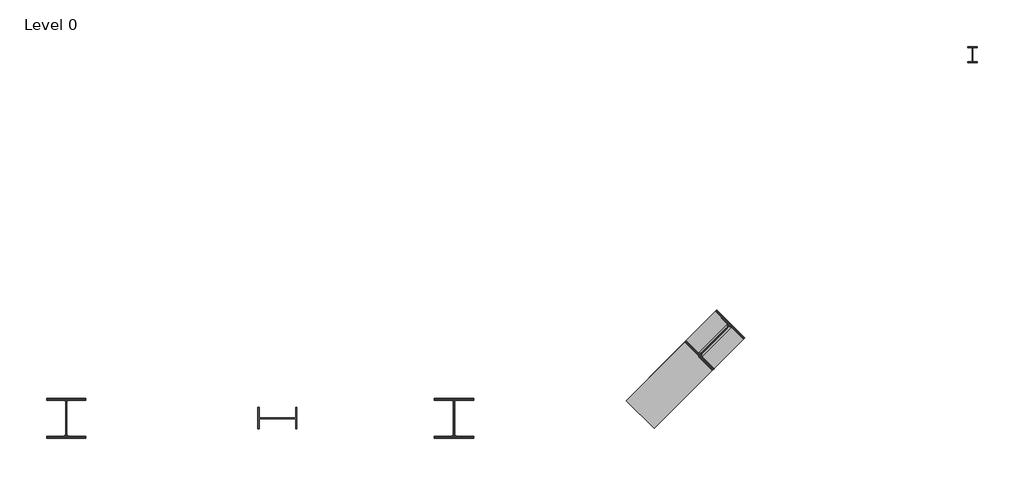
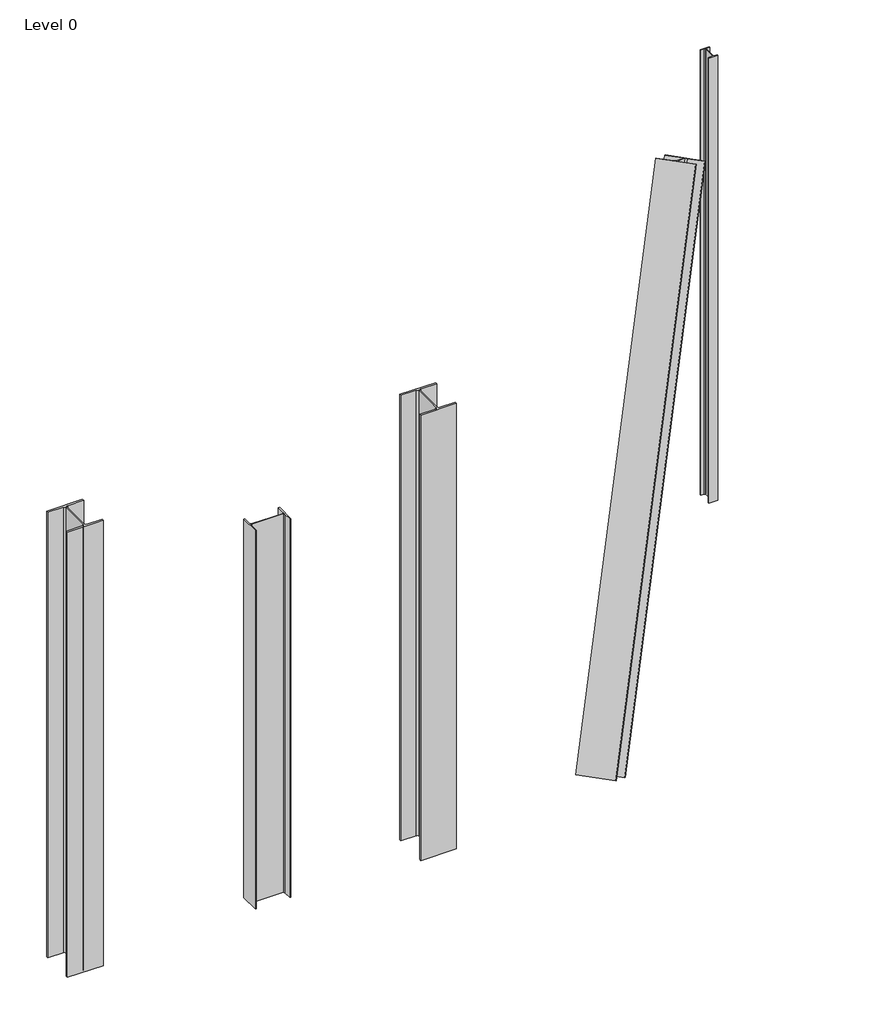
# One storey: 4 columns, 1 member.
"""IFC4 building model written with IfcOpenShell, lengths in millimetres."""

import ifcopenshell
import ifcopenshell.guid

model = None  # the IFC model being written
_history = None  # IfcOwnerHistory: only IFC2X3 demands one
_inside = {}  # id of a spatial element -> (the spatial element, [elements in it])
_under = {}  # id of a project, library or spatial element -> (it, [spatial elements below it])
_declared = {}  # id of a project -> (the project, [libraries it declares])
_typed = {}  # id of a type object -> (the type object, [elements of that type])
_made_of = {}  # id of a material, layer set ... -> (it, [elements and type objects made of it])


def new_model(schema):
    """Start an empty IFC model of exactly this schema.

    Asked for "IFC4X3", IfcOpenShell would pick the latest addendum, in which some entities
    have other attributes; the version numbers below select the first issue.
    IFC2X3 requires an IfcOwnerHistory on every rooted entity: one is made here for all.
    """
    global model, _history
    if schema == "IFC4X3":
        model = ifcopenshell.file(schema_version=(4, 3, 0, 0))
    else:
        model = ifcopenshell.file(schema=schema)
    _inside.clear()
    _under.clear()
    _declared.clear()
    _typed.clear()
    _made_of.clear()
    _history = None
    if model.schema == "IFC2X3":
        org = make("IfcOrganization", Name="unknown")
        user = make(
            "IfcPersonAndOrganization",
            ThePerson=make("IfcPerson", FamilyName="unknown"),
            TheOrganization=org,
        )
        app = make(
            "IfcApplication",
            ApplicationDeveloper=org,
            Version="unknown",
            ApplicationFullName="unknown",
            ApplicationIdentifier="unknown",
        )
        _history = make(
            "IfcOwnerHistory",
            OwningUser=user,
            OwningApplication=app,
            ChangeAction="ADDED",
            CreationDate=0,
        )
    return model


def make(cls, **values):
    """One entity of the class cls with the attributes given. An attribute that is None is left unset."""
    return model.create_entity(
        cls, **{name: value for name, value in values.items() if value is not None}
    )


def rooted(cls, **values):
    """An entity with a GlobalId (a new one), such as an element, a storey or a relation."""
    return make(cls, GlobalId=ifcopenshell.guid.new(), OwnerHistory=_history, **values)


def si_unit(unit_type, name, prefix=None):
    """IfcSIUnit, for example si_unit("LENGTHUNIT", "METRE", prefix="MILLI")."""
    return make("IfcSIUnit", UnitType=unit_type, Prefix=prefix, Name=name)


def assignment(units):
    """IfcUnitAssignment: the units of a project."""
    return None if units is None else make("IfcUnitAssignment", Units=units)


def point(xyz):
    """IfcCartesianPoint."""
    return None if xyz is None else make("IfcCartesianPoint", Coordinates=xyz)


def direction(xyz):
    """IfcDirection."""
    return None if xyz is None else make("IfcDirection", DirectionRatios=xyz)


def frame(location, z_axis=None, x_axis=None):
    """IfcAxis2Placement3D, a coordinate frame: its origin and axes. An axis left out is left unset."""
    return make(
        "IfcAxis2Placement3D",
        Location=point(location),
        Axis=direction(z_axis),
        RefDirection=direction(x_axis),
    )


def frame_2d(location, x_axis=None):
    """IfcAxis2Placement2D, a coordinate frame in the plane: its origin and x axis."""
    return make(
        "IfcAxis2Placement2D", Location=point(location), RefDirection=direction(x_axis)
    )


def origin():
    """The frame at (0, 0, 0) with its axes left unset."""
    return frame((0.0, 0.0, 0.0))


def origin_with_axes():
    """The frame at (0, 0, 0) with the z axis (0, 0, 1) and the x axis (1, 0, 0) written out."""
    return frame((0.0, 0.0, 0.0), z_axis=(0.0, 0.0, 1.0), x_axis=(1.0, 0.0, 0.0))


def place(relative_to, where):
    """IfcLocalPlacement: puts the frame where relative to a parent placement (None: the world)."""
    return make(
        "IfcLocalPlacement", PlacementRelTo=relative_to, RelativePlacement=where
    )


def context(
    kind, dimensions, precision=None, world=None, true_north=None, identifier=None
):
    """IfcGeometricRepresentationContext, for example the 3D "Model" context."""
    return make(
        "IfcGeometricRepresentationContext",
        ContextIdentifier=identifier,
        ContextType=kind,
        CoordinateSpaceDimension=dimensions,
        Precision=precision,
        WorldCoordinateSystem=world,
        TrueNorth=true_north,
    )


def project(units=None, contexts=None):
    """IfcProject with its units and contexts."""
    return rooted(
        "IfcProject",
        Name="project",
        RepresentationContexts=contexts,
        UnitsInContext=assignment(units),
    )


def spatial(cls, under=None, at=None, **own):
    """A site, building, storey or space (cls), placed at a placement, below another one or the project."""
    s = rooted(cls, ObjectPlacement=at, **own)
    if under is not None:
        _under.setdefault(under.id(), (under, []))[1].append(s)
    return s


def polyline(points):
    """IfcPolyline through the points."""
    return make("IfcPolyline", Points=[point(p) for p in points])


def circle_curve(where, radius):
    """IfcCircle in the frame where."""
    return make("IfcCircle", Position=where, Radius=radius)


def trimmed(basis, trim1, trim2, sense, master):
    """IfcTrimmedCurve: the piece of a basis curve between two trims."""
    return make(
        "IfcTrimmedCurve",
        BasisCurve=basis,
        Trim1=trim1,
        Trim2=trim2,
        SenseAgreement=sense,
        MasterRepresentation=master,
    )


def segment(curve, same_sense, transition):
    """IfcCompositeCurveSegment."""
    return make(
        "IfcCompositeCurveSegment",
        Transition=transition,
        SameSense=same_sense,
        ParentCurve=curve,
    )


def composite_curve(segments, self_intersect=None):
    """IfcCompositeCurve: segments joined end to end."""
    return make("IfcCompositeCurve", Segments=segments, SelfIntersect=self_intersect)


def outline(outer, holes=None, kind="AREA"):
    """IfcArbitraryClosedProfileDef: a profile drawn as a closed curve; with holes, ...WithVoids."""
    if holes is None:
        return make("IfcArbitraryClosedProfileDef", ProfileType=kind, OuterCurve=outer)
    return make(
        "IfcArbitraryProfileDefWithVoids",
        ProfileType=kind,
        OuterCurve=outer,
        InnerCurves=holes,
    )


def extrude(swept, where, along, depth):
    """IfcExtrudedAreaSolid: the profile swept, set in the frame where, extruded along a direction by depth."""
    return make(
        "IfcExtrudedAreaSolid",
        SweptArea=swept,
        Position=where,
        ExtrudedDirection=direction(along),
        Depth=depth,
    )


def shape(context_of_items, identifier, shape_type, items):
    """IfcShapeRepresentation: the items that make up one representation, for example the "Body"."""
    return make(
        "IfcShapeRepresentation",
        ContextOfItems=context_of_items,
        RepresentationIdentifier=identifier,
        RepresentationType=shape_type,
        Items=items,
    )


def source(mapping_origin, context_of_items, identifier, shape_type, items):
    """IfcRepresentationMap: a shape defined once, which mapped items show again and again."""
    return make(
        "IfcRepresentationMap",
        MappingOrigin=mapping_origin,
        MappedRepresentation=shape(context_of_items, identifier, shape_type, items),
    )


def transform(
    local_origin,
    x_axis=None,
    y_axis=None,
    z_axis=None,
    scale=None,
    scale2=None,
    scale3=None,
    uniform=True,
):
    """IfcCartesianTransformationOperator3D, or its non-uniform kind. x_axis, y_axis, z_axis: its Axis1, 2, 3."""
    if uniform:
        return make(
            "IfcCartesianTransformationOperator3D",
            Axis1=direction(x_axis),
            Axis2=direction(y_axis),
            LocalOrigin=point(local_origin),
            Scale=scale,
            Axis3=direction(z_axis),
        )
    return make(
        "IfcCartesianTransformationOperator3DnonUniform",
        Axis1=direction(x_axis),
        Axis2=direction(y_axis),
        LocalOrigin=point(local_origin),
        Scale=scale,
        Axis3=direction(z_axis),
        Scale2=scale2,
        Scale3=scale3,
    )


def mapped(mapping_source, mapping_target):
    """IfcMappedItem: shows the shape of a source again, moved by a transform."""
    return make(
        "IfcMappedItem", MappingSource=mapping_source, MappingTarget=mapping_target
    )


def made_of(thing, what):
    """Note that an element or type object is made of a material, layer set ...; save() writes the relation."""
    if what is not None:
        _made_of.setdefault(what.id(), (what, []))[1].append(thing)
    return thing


def element(
    cls,
    number,
    at=None,
    inside=None,
    cuts=None,
    type_object=None,
    material=None,
    context=None,
    identifier="Body",
    shape_type=None,
    held_by="IfcProductDefinitionShape",
    body=None,
    shapes=None,
    **own,
):
    """One element of the class cls, such as IfcWall. Its Tag is "e" and its number.

    at: its placement. inside: the storey or other place that contains it. cuts: it is an
    opening in that element (IfcRelVoidsElement). A single representation is given by context,
    identifier, shape_type and body (its items); several are given by shapes. held_by: the class
    of the entity that holds the representations. save() writes the other relations.
    """
    e = rooted(cls, Tag="e%d" % number, ObjectPlacement=at, **own)
    if body is not None:
        shapes = [shape(context, identifier, shape_type, body)]
    if shapes is not None:
        e.Representation = make(held_by, Representations=shapes)
    if inside is not None:
        _inside.setdefault(inside.id(), (inside, []))[1].append(e)
    if cuts is not None:
        rooted(
            "IfcRelVoidsElement", RelatingBuildingElement=cuts, RelatedOpeningElement=e
        )
    if type_object is not None:
        _typed.setdefault(type_object.id(), (type_object, []))[1].append(e)
    return made_of(e, material)


def aggregate(whole, parts):
    """IfcRelAggregates: a whole, such as a stair, and the parts it consists of."""
    return rooted("IfcRelAggregates", RelatingObject=whole, RelatedObjects=parts)


def save(model, path):
    """Write the relations noted so far, then the file.

    IfcRelAggregates (storeys below a building ...), IfcRelContainedInSpatialStructure (elements
    in a storey), IfcRelDefinesByType, IfcRelAssociatesMaterial and IfcRelDeclares: one each for
    every whole, place, type object, material and project.
    """
    for whole, parts in _under.values():
        aggregate(whole, parts)
    for where, things in _inside.values():
        rooted(
            "IfcRelContainedInSpatialStructure",
            RelatedElements=things,
            RelatingStructure=where,
        )
    for kind, things in _typed.values():
        rooted("IfcRelDefinesByType", RelatedObjects=things, RelatingType=kind)
    for what, things in _made_of.values():
        rooted("IfcRelAssociatesMaterial", RelatedObjects=things, RelatingMaterial=what)
    for by, libraries in _declared.values():
        rooted("IfcRelDeclares", RelatingContext=by, RelatedDefinitions=libraries)
    model.write(path)


def ub_universal_beams_column_ub127x76x13_3e05bf5d(model_context):
    return source(origin(), model_context, "Body", "SweptSolid", [
        extrude(outline(composite_curve([segment(polyline([(38.0, 63.5), (38.0, 55.9), (9.6, 55.9)]), True, "CONTINUOUS"), segment(trimmed(circle_curve(frame_2d((9.6, 48.3)), 7.6), [point((9.6, 55.9))], [point((2.0, 48.3))], True, "CARTESIAN"), True, "CONTINUOUS"), segment(polyline([(2.0, 48.3), (2.0, -48.3)]), True, "CONTINUOUS"), segment(trimmed(circle_curve(frame_2d((9.6, -48.3)), 7.6), [point((2.0, -48.3))], [point((9.6, -55.9))], True, "CARTESIAN"), True, "CONTINUOUS"), segment(polyline([(9.6, -55.9), (38.0, -55.9), (38.0, -63.5), (-38.0, -63.5), (-38.0, -55.9), (-9.6, -55.9)]), True, "CONTINUOUS"), segment(trimmed(circle_curve(frame_2d((-9.6, -48.3)), 7.6), [point((-9.6, -55.9))], [point((-2.0, -48.3))], True, "CARTESIAN"), True, "CONTINUOUS"), segment(polyline([(-2.0, -48.3), (-2.0, 48.3)]), True, "CONTINUOUS"), segment(trimmed(circle_curve(frame_2d((-9.6, 48.3)), 7.6), [point((-2.0, 48.3))], [point((-9.6, 55.9))], True, "CARTESIAN"), True, "CONTINUOUS"), segment(polyline([(-9.6, 55.9), (-38.0, 55.9), (-38.0, 63.5), (38.0, 63.5)]), True, "CONTINUOUS")], self_intersect=False)), origin_with_axes(), (0.0, 0.0, 1.0), 4000.0),
    ])


def uc_universal_columns_column_uc305x305x97_9aa56e74(model_context):
    return source(origin(), model_context, "Body", "SweptSolid", [
        extrude(outline(composite_curve([segment(polyline([(152.65, 153.95), (152.65, 138.55), (20.15, 138.55)]), True, "CONTINUOUS"), segment(trimmed(circle_curve(frame_2d((20.15, 123.35)), 15.2), [point((20.15, 138.55))], [point((4.95, 123.35))], True, "CARTESIAN"), True, "CONTINUOUS"), segment(polyline([(4.95, 123.35), (4.95, -123.35)]), True, "CONTINUOUS"), segment(trimmed(circle_curve(frame_2d((20.15, -123.35)), 15.2), [point((4.95, -123.35))], [point((20.15, -138.55))], True, "CARTESIAN"), True, "CONTINUOUS"), segment(polyline([(20.15, -138.55), (152.65, -138.55), (152.65, -153.95), (-152.65, -153.95), (-152.65, -138.55), (-20.15, -138.55)]), True, "CONTINUOUS"), segment(trimmed(circle_curve(frame_2d((-20.15, -123.35)), 15.2), [point((-20.15, -138.55))], [point((-4.95, -123.35))], True, "CARTESIAN"), True, "CONTINUOUS"), segment(polyline([(-4.95, -123.35), (-4.95, 123.35)]), True, "CONTINUOUS"), segment(trimmed(circle_curve(frame_2d((-20.15, 123.35)), 15.2), [point((-4.95, 123.35))], [point((-20.15, 138.55))], True, "CARTESIAN"), True, "CONTINUOUS"), segment(polyline([(-20.15, 138.55), (-152.65, 138.55), (-152.65, 153.95), (152.65, 153.95)]), True, "CONTINUOUS")], self_intersect=False)), origin_with_axes(), (0.0, 0.0, 1.0), 4000.0),
    ])


def uc_universal_columns_column_uc305x305x97_7d345059(model_context):
    return source(origin(), model_context, "Body", "SweptSolid", [
        extrude(outline(composite_curve([segment(polyline([(152.65, -153.95), (-152.65, -153.95), (-152.65, -138.55), (-20.15, -138.55)]), True, "CONTINUOUS"), segment(trimmed(circle_curve(frame_2d((-20.15, -123.35)), 15.2), [point((-20.15, -138.55))], [point((-4.95, -123.35))], True, "CARTESIAN"), True, "CONTINUOUS"), segment(polyline([(-4.95, -123.35), (-4.95, 123.35)]), True, "CONTINUOUS"), segment(trimmed(circle_curve(frame_2d((-20.15, 123.35)), 15.2), [point((-4.95, 123.35))], [point((-20.15, 138.55))], True, "CARTESIAN"), True, "CONTINUOUS"), segment(polyline([(-20.15, 138.55), (-152.65, 138.55), (-152.65, 153.95), (152.65, 153.95), (152.65, 138.55), (20.15, 138.55)]), True, "CONTINUOUS"), segment(trimmed(circle_curve(frame_2d((20.15, 123.35)), 15.2), [point((20.15, 138.55))], [point((4.95, 123.35))], True, "CARTESIAN"), True, "CONTINUOUS"), segment(polyline([(4.95, 123.35), (4.95, -123.35)]), True, "CONTINUOUS"), segment(trimmed(circle_curve(frame_2d((20.15, -123.35)), 15.2), [point((4.95, -123.35))], [point((20.15, -138.55))], True, "CARTESIAN"), True, "CONTINUOUS"), segment(polyline([(20.15, -138.55), (152.65, -138.55), (152.65, -153.95)]), True, "CONTINUOUS")], self_intersect=False)), origin_with_axes(), (0.0, 0.0, 1.0), 4000.0),
    ])


def ub_universal_beams_ub305x165x40_ae602ee7(model_context):
    return source(origin(), model_context, "Body", "SweptSolid", [
        extrude(outline(composite_curve([segment(polyline([(82.5, -141.5), (82.5, -151.7), (-82.5, -151.7), (-82.5, -141.5), (-11.9, -141.5)]), True, "CONTINUOUS"), segment(trimmed(circle_curve(frame_2d((-11.9, -132.6)), 8.9), [point((-11.9, -141.5))], [point((-3.0, -132.6))], True, "CARTESIAN"), True, "CONTINUOUS"), segment(polyline([(-3.0, -132.6), (-3.0, 132.6)]), True, "CONTINUOUS"), segment(trimmed(circle_curve(frame_2d((-11.9, 132.6)), 8.9), [point((-3.0, 132.6))], [point((-11.9, 141.5))], True, "CARTESIAN"), True, "CONTINUOUS"), segment(polyline([(-11.9, 141.5), (-82.5, 141.5), (-82.5, 151.7), (82.5, 151.7), (82.5, 141.5), (11.9, 141.5)]), True, "CONTINUOUS"), segment(trimmed(circle_curve(frame_2d((11.9, 132.6)), 8.9), [point((11.9, 141.5))], [point((3.0, 132.6))], True, "CARTESIAN"), True, "CONTINUOUS"), segment(polyline([(3.0, 132.6), (3.0, -132.6)]), True, "CONTINUOUS"), segment(trimmed(circle_curve(frame_2d((11.9, -132.6)), 8.9), [point((3.0, -132.6))], [point((11.9, -141.5))], True, "CARTESIAN"), True, "CONTINUOUS"), segment(polyline([(11.9, -141.5), (82.5, -141.5)]), True, "CONTINUOUS")], self_intersect=False)), frame((-1700.0, 0.0, 0.0), z_axis=(1.0, 0.0, 0.0), x_axis=(0.0, 1.0, 0.0)), (0.0, 0.0, 1.0), 3400.0),
    ])


model = new_model("IFC4")

# Units and contexts
model_context = context("Model", 3, world=origin())
ifc_project = project(units=[si_unit("LENGTHUNIT", "METRE", prefix="MILLI")], contexts=[model_context])

# Site, building, storey
site = spatial("IfcSite", under=ifc_project)
building = spatial("IfcBuilding", under=site)
storey = spatial("IfcBuildingStorey", under=building, Name="Level 0", Elevation=0.0)

# Columns
placement = place(None, origin())
ub_universal_beams_column_ub127x76x13_shape = ub_universal_beams_column_ub127x76x13_3e05bf5d(model_context)
element("IfcColumn", 1, ObjectType="UB-Universal Beams-Column : UB127x76x13", at=placement, inside=storey, context=model_context, shape_type="MappedRepresentation", body=[
    mapped(ub_universal_beams_column_ub127x76x13_shape, transform((8826.7923839, 3472.3264639, 0.0), x_axis=(1.0, 0.0, 0.0), y_axis=(0.0, 1.0, 0.0), z_axis=(0.0, 0.0, 1.0))),
])
element("IfcColumn", 2, ObjectType="UC-Universal Columns-Column : UC305x305x97", at=placement, inside=storey, context=model_context, shape_type="SweptSolid", body=[
    extrude(outline(composite_curve([segment(polyline([(305.3, 0.0), (305.2999999, -15.4), (172.7999999, -15.4)]), True, "CONTINUOUS"), segment(trimmed(circle_curve(frame_2d((172.7999999, -30.6)), 15.2), [point((172.7999999, -15.4))], [point((157.5999999, -30.6))], True, "CARTESIAN"), True, "CONTINUOUS"), segment(polyline([(157.5999999, -30.6), (157.6, -277.3)]), True, "CONTINUOUS"), segment(trimmed(circle_curve(frame_2d((172.7999999, -277.2999999)), 15.2), [point((157.6, -277.3))], [point((172.7999999, -292.5))], True, "CARTESIAN"), True, "CONTINUOUS"), segment(polyline([(172.7999999, -292.5), (305.3, -292.5), (305.2999999, -307.9), (-1e-07, -307.9), (0.0, -292.5), (132.5, -292.5)]), True, "CONTINUOUS"), segment(trimmed(circle_curve(frame_2d((132.5, -277.3)), 15.2), [point((132.5, -292.5))], [point((147.7, -277.2999999))], True, "CARTESIAN"), True, "CONTINUOUS"), segment(polyline([(147.7, -277.2999999), (147.7, -30.6)]), True, "CONTINUOUS"), segment(trimmed(circle_curve(frame_2d((132.4999999, -30.6)), 15.2), [point((147.7, -30.6))], [point((132.5, -15.4))], True, "CARTESIAN"), True, "CONTINUOUS"), segment(polyline([(132.5, -15.4), (0.0, -15.4), (0.0, 0.0), (305.3, 0.0)]), True, "CONTINUOUS")], self_intersect=False)), frame((6362.6217623, 576.3964418, 76.0232991), z_axis=(0.34918213922193536, 0.3491821392219347, 0.8695652173913044), x_axis=(-0.7071067811865468, 0.7071067811865482, 0.0)), (0.0, 0.0, 1.0), 4600.0),
])
uc_universal_columns_column_uc305x305x97_shape = uc_universal_columns_column_uc305x305x97_9aa56e74(model_context)
element("IfcColumn", 3, ObjectType="UC-Universal Columns-Column : UC305x305x97", at=placement, inside=storey, context=model_context, shape_type="MappedRepresentation", body=[
    mapped(uc_universal_columns_column_uc305x305x97_shape, transform((1813.0340314, 656.2752041, 0.0), x_axis=(1.0, 0.0, 0.0), y_axis=(0.0, 1.0, 0.0), z_axis=(0.0, 0.0, 1.0))),
])
uc_universal_columns_column_uc305x305x97_2_shape = uc_universal_columns_column_uc305x305x97_7d345059(model_context)
element("IfcColumn", 4, ObjectType="UC-Universal Columns-Column : UC305x305x97", at=placement, inside=storey, context=model_context, shape_type="MappedRepresentation", body=[
    mapped(uc_universal_columns_column_uc305x305x97_2_shape, transform((4813.0340314, 656.2752041, 0.0), x_axis=(-1.0, 0.0, 0.0), y_axis=(0.0, -1.0, 0.0), z_axis=(0.0, 0.0, 1.0))),
])

# Member
ub_universal_beams_ub305x165x40_shape = ub_universal_beams_ub305x165x40_ae602ee7(model_context)
element("IfcMember", 5, ObjectType="UB-Universal Beams : UB305x165x40", at=placement, inside=storey, context=model_context, shape_type="MappedRepresentation", body=[
    mapped(ub_universal_beams_ub305x165x40_shape, transform((3446.7055137, 656.2752041, 1700.0), x_axis=(0.0, 0.0, 1.0), y_axis=(0.0, 1.0, 0.0), z_axis=(-1.0, 0.0, 0.0))),
])

save(model, "model.ifc")

# Revit data of these elements
# Project information
#   Project Issue Date = "Issue Date"
#   Project Status = "Project Status"
#   Client Name = "Owner"
#   Project Address = "Enter address here"
#   Project Name = "Project Name"
#   Project Number = "Project Number"
# Type "UB-Universal Beams-Column : UB127x76x13"
#   Section Name Key = "UB127X76X13"
#   Width = 7.6 cm
#   Web Thickness = 0.4 cm
#   Web Fillet = 0.76 cm
#   Warping Constant = 2000.0 cm⁶
#   Torsional Moment of Inertia = 2.85 cm⁴
#   Section Area = 16.5 cm²
#   Plastic Modulus weak axis = 22.6 cm³
#   Plastic Modulus strong axis = 84.2 cm³
#   Nominal Weight = 13.00 kgf/m
#   Moment of Inertia weak axis = 55.70 cm⁴
#   Moment of Inertia strong axis = 473.00 cm⁴
#   Height = 12.7 cm
#   Flange Thickness = 0.76 cm
#   Elastic Modulus weak axis = 14.7 cm³
#   Elastic Modulus strong axis = 74.6 cm³
#   Centroid Vertical = 6.35 cm
#   Centroid Horizontal = 3.8 cm
#   Bolt Spacing = 4.0 cm
#   Structural Material [instance default] = Metal - Steel 43-275
#   Type Comments = ""
#   Assembly Code = ""
# Type "UC-Universal Columns-Column : UC305x305x97"
#   Section Name Key = "UC305x305x97"
#   Width = 30.53 cm
#   Web Thickness = 0.99 cm
#   Web Fillet = 1.52 cm
#   Warping Constant = 1560000.0 cm⁶
#   Torsional Moment of Inertia = 91.20 cm⁴
#   Section Area = 123.0 cm²
#   Plastic Modulus weak axis = 726.0 cm³
#   Plastic Modulus strong axis = 1592.0 cm³
#   Nominal Weight = 96.8996 kgf/m
#   Moment of Inertia weak axis = 7308.00 cm⁴
#   Moment of Inertia strong axis = 22249.00 cm⁴
#   Height = 30.79 cm
#   Flange Thickness = 1.54 cm
#   Elastic Modulus weak axis = 479.0 cm³
#   Elastic Modulus strong axis = 1445.0 cm³
#   Centroid Vertical = 15.395 cm
#   Centroid Horizontal = 15.265 cm
#   Bolt Spacing = 14.0 cm
#   Structural Material [instance default] = Metal - Steel 43-275
#   Type Comments = ""
#   Assembly Code = ""
# Type "UB-Universal Beams : UB305x165x40"
#   Section Name Key = "UB305X165X40"
#   Width = 16.5 cm
#   Web Thickness = 0.6 cm
#   Web Fillet = 0.89 cm
#   Warping Constant = 164000.0 cm⁶
#   Torsional Moment of Inertia = 14.70 cm⁴
#   Section Area = 51.3 cm²
#   Plastic Modulus weak axis = 142.0 cm³
#   Plastic Modulus strong axis = 623.0 cm³
#   Nominal Weight = 40.2999 kgf/m
#   Moment of Inertia weak axis = 764.00 cm⁴
#   Moment of Inertia strong axis = 8503.00 cm⁴
#   Height = 30.34 cm
#   Flange Thickness = 1.02 cm
#   Elastic Modulus weak axis = 92.6 cm³
#   Elastic Modulus strong axis = 560.0 cm³
#   Centroid Vertical = 15.17 cm
#   Centroid Horizontal = 8.25 cm
#   Bolt Spacing = 9.0 cm
#   Length [instance default] = 1500 mm
#   Structural Material [instance default] = Metal - Steel 43-275
#   Type Comments = ""
#   Assembly Code = ""
# Element 1 (IfcColumn, "UB-Universal Beams-Column : UB127x76x13")
#   Structural Material = Metal - Steel 43-275
#   Phase Created = New Construction
#   Materials on its faces: "Metal - Steel 43-275"
# Elements 2, 4 (IfcColumn, "UC-Universal Columns-Column : UC305x305x97")
#   Structural Material = Metal - Steel 43-275
#   Phase Created = New Construction
#   Materials on its faces: "Metal - Steel 43-275"
# Element 3 (IfcColumn, "UC-Universal Columns-Column : UC305x305x97")
#   Comments = ""
#   Structural Material = Metal - Steel 43-275
#   Phase Created = New Construction
#   Materials on its faces: "Metal - Steel 43-275"
# Element 5 (IfcMember, "UB-Universal Beams : UB305x165x40")
#   Structural Material = Metal - Steel 43-275
#   Phase Created = New Construction
#   Materials on its faces: "Metal - Steel 43-275"
# Materials
#   "Metal - Steel 43-275": class "Metal", colour RGB 247 247 247, transparency 0, Cost = 0
